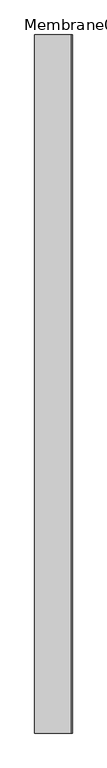
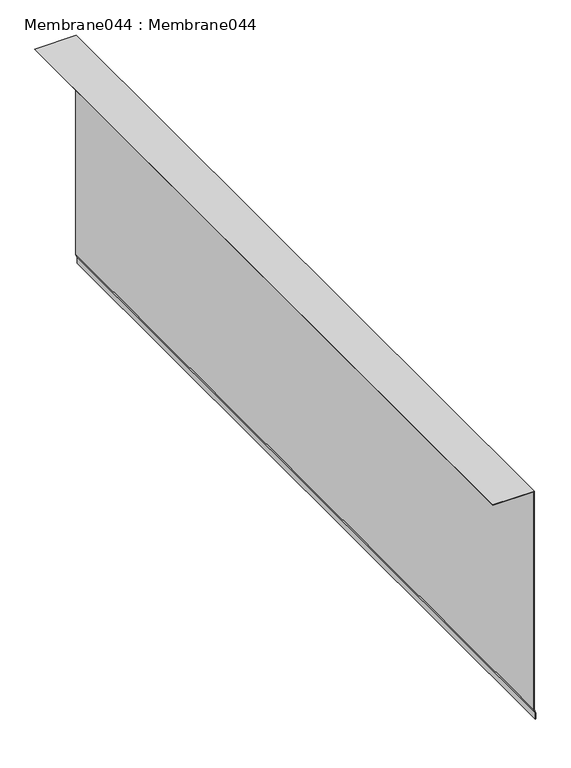
"""IFC4 building model written with IfcOpenShell, lengths in millimetres: proxy geometry, Membrane044 : Membrane044."""

from ifc_helpers import new_model, si_unit, frame, origin, place, context, project, spatial, polyline, outline, extrude, source, transform, mapped, element, save


def membrane044_membrane044_10a2dc38(model_context):
    return source(origin(), model_context, "Body", "SweptSolid", [
        extrude(outline(polyline([(40160.8681333, -9398.2396626), (40159.8681333, -9398.2396626), (40159.8681333, -9295.4978798), (39579.3230707, -9295.4978798), (39568.0978055, -9291.4122174), (39552.6918208, -9291.4122174), (39552.6918208, -9290.4122174), (39568.2741325, -9290.4122174), (39579.4993977, -9294.4978798), (40160.8681333, -9294.4978798), (40160.8681333, -9398.2396626)])), frame((0.0, 7982.1531721, 0.0), z_axis=(0.0, 1.0, 0.0), x_axis=(0.0, 0.0, 1.0)), (0.0, 0.0, 1.0), 2000.0),
    ])


if __name__ == "__main__":
    model = new_model("IFC4")
    model_context = context("Model", 3, world=origin())
    ifc_project = project(units=[si_unit("LENGTHUNIT", "METRE", prefix="MILLI")], contexts=[model_context])
    site = spatial("IfcSite", under=ifc_project)
    building = spatial("IfcBuilding", under=site)
    placement = place(None, origin())
    membrane044_membrane044_shape = membrane044_membrane044_10a2dc38(model_context)
    element("IfcBuildingElementProxy", 1, Name="Membrane044 : Membrane044", ObjectType="Membrane044 : Membrane044", at=placement, inside=building, context=model_context, shape_type="MappedRepresentation", body=[
        mapped(membrane044_membrane044_shape, transform((0.0, 0.0, 0.0), x_axis=(1.0, 0.0, 0.0), y_axis=(0.0, 1.0, 0.0), z_axis=(0.0, 0.0, 1.0))),
    ])
    save(model, "model.ifc")

# Revit data of these elements
# Type "Membrane044 : Membrane044"
#   NameOverride = "Membrane044"
# Element 1 (IfcBuildingElementProxy, "Membrane044 : Membrane044")
#   Materials on its faces: "2 LAYERS NO. 30 ASTM D226 ASPHALT SATURATED ORGANIC FELT"
# Materials
#   "2 LAYERS NO. 30 ASTM D226 ASPHALT SATURATED ORGANIC FELT": class "Unassigned", colour RGB 46 171 0, transparency 0
